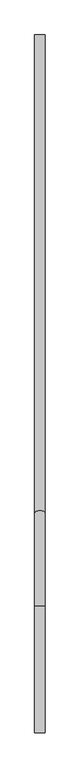
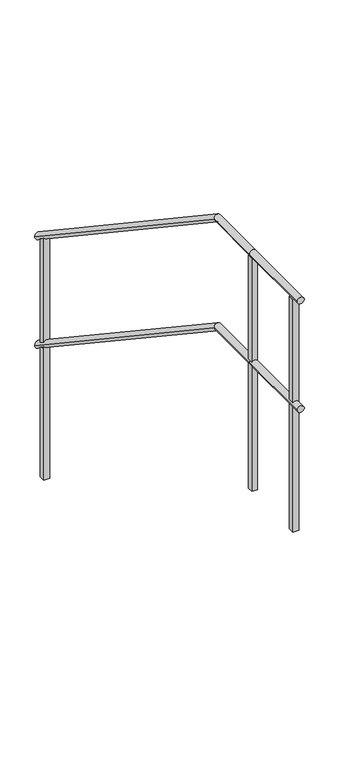
"""IFC4 building model written with IfcOpenShell, lengths in millimetres: railing geometry."""

from ifc_helpers import new_model, si_unit, frame, origin, place, context, project, spatial, polyline, circle_curve, ellipse_curve, outline, extrude, source, transform, mapped, element, save
from ifc_brep_helpers import plane_surface, cylinder_surface, advanced_brep


def railing_d4b76e20(model_context):
    return source(origin(), model_context, "Body", "SolidModel", [
        advanced_brep(
        [(12192.5845799, 439.5208589, 9334.9618634), (12162.5845799, 439.5208589, 9334.9618634), (12192.5845799, 799.5208589, 9334.9618634), (12162.5845799, 799.5208589, 9334.9618634)],
        [
            (0, 1, circle_curve(frame((12177.5845799, 439.5208589, 9334.9618634), z_axis=(0.0, -1.0, 0.0), x_axis=(-1.0, 0.0, 0.0)), 15.0)),
            (1, 0, circle_curve(frame((12177.5845799, 439.5208589, 9334.9618634), z_axis=(0.0, -1.0, 0.0), x_axis=(-1.0, 0.0, 0.0)), 15.0)),
            (2, 3, circle_curve(frame((12177.5845799, 799.5208589, 9334.9618634), z_axis=(0.0, 1.0, 0.0), x_axis=(-1.0, 0.0, 0.0)), 15.0)),
            (3, 2, circle_curve(frame((12177.5845799, 799.5208589, 9334.9618634), z_axis=(0.0, 1.0, 0.0), x_axis=(-1.0, 0.0, 0.0)), 15.0)),
            (1, 3),
            (2, 0),
        ],
        [
            plane_surface(frame((12177.5845799, 439.5208589, 9349.9618634), z_axis=(0.0, -1.0, 0.0), x_axis=(0.0, 0.0, 1.0))),
            plane_surface(frame((12177.5845799, 799.5208589, 9349.9618634), z_axis=(0.0, 1.0, 0.0), x_axis=(0.0, 0.0, 1.0))),
            cylinder_surface(frame((12177.5845799, 439.5208589, 9334.9618634), z_axis=(0.0, -1.0, 0.0), x_axis=(-1.0, 0.0, 0.0)), 15.0),
        ],
        [
            (0, [[1, 2]]),
            (1, [[3, 4]]),
            (2, [[-2, 5, -3, 6]]),
            (2, [[-1, -6, -4, -5]]),
        ],
    ),
        advanced_brep(
        [(12192.5845799, 799.5208589, 9334.9618634), (12162.5845799, 799.5208589, 9334.9618634), (12162.5845799, 1064.9792243, 9334.9618634), (12192.5845799, 1064.9792243, 9334.9618634), (12192.5845799, 2419.5208589, 8431.934107), (12162.5845799, 2419.5208589, 8431.934107)],
        [
            (0, 1, circle_curve(frame((12177.5845799, 799.5208589, 9334.9618634), z_axis=(0.0, -1.0, 0.0), x_axis=(-1.0, 0.0, 0.0)), 15.0)),
            (1, 0, circle_curve(frame((12177.5845799, 799.5208589, 9334.9618634), z_axis=(0.0, -1.0, 0.0), x_axis=(-1.0, 0.0, 0.0)), 15.0)),
            (1, 2),
            (2, 3, ellipse_curve(frame((12177.5845799, 1064.9792243, 9334.9618634), z_axis=(0.0, -0.9570920264890528, 0.28978414868843017), x_axis=(0.0, -0.2897841486884305, -0.9570920264890528)), 15.6724741, 15.0)),
            (3, 0),
            (3, 2, ellipse_curve(frame((12177.5845799, 1064.9792243, 9334.9618634), z_axis=(0.0, -0.9570920264890528, 0.28978414868843017), x_axis=(0.0, -0.2897841486884305, -0.9570920264890528)), 15.6724741, 15.0)),
            (4, 5, ellipse_curve(frame((12177.5845799, 2419.5208589, 8431.934107), z_axis=(0.0, 1.0, 0.0), x_axis=(0.0, 0.0, 1.0)), 18.0277564, 15.0)),
            (5, 4, ellipse_curve(frame((12177.5845799, 2419.5208589, 8431.934107), z_axis=(0.0, 1.0, 0.0), x_axis=(0.0, 0.0, 1.0)), 18.0277564, 15.0)),
            (2, 5),
            (4, 3),
        ],
        [
            plane_surface(frame((12177.5845799, 799.5208589, 9349.9618634), z_axis=(0.0, -1.0, 0.0), x_axis=(0.0, 0.0, 1.0))),
            cylinder_surface(frame((12177.5845799, 799.5208589, 9334.9618634), z_axis=(0.0, -1.0, 0.0), x_axis=(-1.0, 0.0, 0.0)), 15.0),
            plane_surface(frame((12177.5845799, 2419.5208589, 8449.9618634), z_axis=(0.0, 1.0, 0.0), x_axis=(0.0, 0.0, 1.0))),
            cylinder_surface(frame((12177.5845799, 1061.2003559, 9337.481109), z_axis=(0.0, -0.8320502943378436, 0.5547001962252293), x_axis=(-1.0, 0.0, 0.0)), 15.0),
        ],
        [
            (0, [[1, 2]]),
            (1, [[-2, 3, 4, 5]]),
            (1, [[-1, -5, 6, -3]]),
            (2, [[7, 8]]),
            (3, [[-4, 9, -7, 10]]),
            (3, [[-6, -10, -8, -9]]),
        ],
    ),
        advanced_brep(
        [(12192.5845799, 439.5208589, 9834.9618634), (12162.5845799, 439.5208589, 9834.9618634), (12192.5845799, 799.5208589, 9834.9618634), (12162.5845799, 799.5208589, 9834.9618634)],
        [
            (0, 1, circle_curve(frame((12177.5845799, 439.5208589, 9834.9618634), z_axis=(0.0, -1.0, 0.0), x_axis=(-1.0, 0.0, 0.0)), 15.0)),
            (1, 0, circle_curve(frame((12177.5845799, 439.5208589, 9834.9618634), z_axis=(0.0, -1.0, 0.0), x_axis=(-1.0, 0.0, 0.0)), 15.0)),
            (2, 3, circle_curve(frame((12177.5845799, 799.5208589, 9834.9618634), z_axis=(0.0, 1.0, 0.0), x_axis=(-1.0, 0.0, 0.0)), 15.0)),
            (3, 2, circle_curve(frame((12177.5845799, 799.5208589, 9834.9618634), z_axis=(0.0, 1.0, 0.0), x_axis=(-1.0, 0.0, 0.0)), 15.0)),
            (1, 3),
            (2, 0),
        ],
        [
            plane_surface(frame((12177.5845799, 439.5208589, 9849.9618634), z_axis=(0.0, -1.0, 0.0), x_axis=(0.0, 0.0, 1.0))),
            plane_surface(frame((12177.5845799, 799.5208589, 9849.9618634), z_axis=(0.0, 1.0, 0.0), x_axis=(0.0, 0.0, 1.0))),
            cylinder_surface(frame((12177.5845799, 439.5208589, 9834.9618634), z_axis=(0.0, -1.0, 0.0), x_axis=(-1.0, 0.0, 0.0)), 15.0),
        ],
        [
            (0, [[1, 2]]),
            (1, [[3, 4]]),
            (2, [[-2, 5, -3, 6]]),
            (2, [[-1, -6, -4, -5]]),
        ],
    ),
        advanced_brep(
        [(12192.5845799, 799.5208589, 9834.9618634), (12162.5845799, 799.5208589, 9834.9618634), (12162.5845799, 1064.9792243, 9834.9618634), (12192.5845799, 1064.9792243, 9834.9618634), (12192.5845799, 2419.5208589, 8931.934107), (12162.5845799, 2419.5208589, 8931.934107)],
        [
            (0, 1, circle_curve(frame((12177.5845799, 799.5208589, 9834.9618634), z_axis=(0.0, -1.0, 0.0), x_axis=(-1.0, 0.0, 0.0)), 15.0)),
            (1, 0, circle_curve(frame((12177.5845799, 799.5208589, 9834.9618634), z_axis=(0.0, -1.0, 0.0), x_axis=(-1.0, 0.0, 0.0)), 15.0)),
            (1, 2),
            (2, 3, ellipse_curve(frame((12177.5845799, 1064.9792243, 9834.9618634), z_axis=(0.0, -0.9570920264890528, 0.28978414868843017), x_axis=(0.0, -0.2897841486884305, -0.9570920264890528)), 15.6724741, 15.0)),
            (3, 0),
            (3, 2, ellipse_curve(frame((12177.5845799, 1064.9792243, 9834.9618634), z_axis=(0.0, -0.9570920264890528, 0.28978414868843017), x_axis=(0.0, -0.2897841486884305, -0.9570920264890528)), 15.6724741, 15.0)),
            (4, 5, ellipse_curve(frame((12177.5845799, 2419.5208589, 8931.934107), z_axis=(0.0, 1.0, 0.0), x_axis=(0.0, 0.0, 1.0)), 18.0277564, 15.0)),
            (5, 4, ellipse_curve(frame((12177.5845799, 2419.5208589, 8931.934107), z_axis=(0.0, 1.0, 0.0), x_axis=(0.0, 0.0, 1.0)), 18.0277564, 15.0)),
            (2, 5),
            (4, 3),
        ],
        [
            plane_surface(frame((12177.5845799, 799.5208589, 9849.9618634), z_axis=(0.0, -1.0, 0.0), x_axis=(0.0, 0.0, 1.0))),
            cylinder_surface(frame((12177.5845799, 799.5208589, 9834.9618634), z_axis=(0.0, -1.0, 0.0), x_axis=(-1.0, 0.0, 0.0)), 15.0),
            plane_surface(frame((12177.5845799, 2419.5208589, 8949.9618634), z_axis=(0.0, 1.0, 0.0), x_axis=(0.0, 0.0, 1.0))),
            cylinder_surface(frame((12177.5845799, 1061.2003559, 9837.481109), z_axis=(0.0, -0.8320502943378436, 0.5547001962252293), x_axis=(-1.0, 0.0, 0.0)), 15.0),
        ],
        [
            (0, [[1, 2]]),
            (1, [[-2, 3, 4, 5]]),
            (1, [[-1, -5, 6, -3]]),
            (2, [[7, 8]]),
            (3, [[-4, 9, -7, 10]]),
            (3, [[-6, -10, -8, -9]]),
        ],
    ),
        extrude(outline(polyline([(12165.0845799, 787.0208589), (12165.0845799, 812.0208589), (12190.0845799, 812.0208589), (12190.0845799, 787.0208589), (12165.0845799, 787.0208589)])), frame((0.0, 0.0, 8749.9618634), z_axis=(0.0, 0.0, 1.0), x_axis=(1.0, 0.0, 0.0)), (0.0, 0.0, 1.0), 1070.0),
        extrude(outline(polyline([(2357.0208589, 8961.62853), (2382.0208589, 8944.9618634), (2382.0208589, 7849.9618634), (2357.0208589, 7849.9618634), (2357.0208589, 8961.62853)])), frame((12165.0845799, 0.0, 0.0), z_axis=(1.0, 0.0, 0.0), x_axis=(0.0, 1.0, 0.0)), (0.0, 0.0, 1.0), 25.0),
        extrude(outline(polyline([(12165.0845799, 477.0208589), (12165.0845799, 502.0208589), (12190.0845799, 502.0208589), (12190.0845799, 477.0208589), (12165.0845799, 477.0208589)])), frame((0.0, 0.0, 8749.9618634), z_axis=(0.0, 0.0, 1.0), x_axis=(1.0, 0.0, 0.0)), (0.0, 0.0, 1.0), 1070.0),
    ])


if __name__ == "__main__":
    model = new_model("IFC4")
    model_context = context("Model", 3, world=origin())
    ifc_project = project(units=[si_unit("LENGTHUNIT", "METRE", prefix="MILLI")], contexts=[model_context])
    site = spatial("IfcSite", under=ifc_project)
    building = spatial("IfcBuilding", under=site)
    placement = place(None, origin())
    railing_shape = railing_d4b76e20(model_context)
    element("IfcRailing", 1, at=placement, inside=building, context=model_context, shape_type="MappedRepresentation", body=[
        mapped(railing_shape, transform((0.0, 0.0, 0.0), x_axis=(1.0, 0.0, 0.0), y_axis=(0.0, 1.0, 0.0), z_axis=(0.0, 0.0, 1.0))),
    ])
    save(model, "model.ifc")
